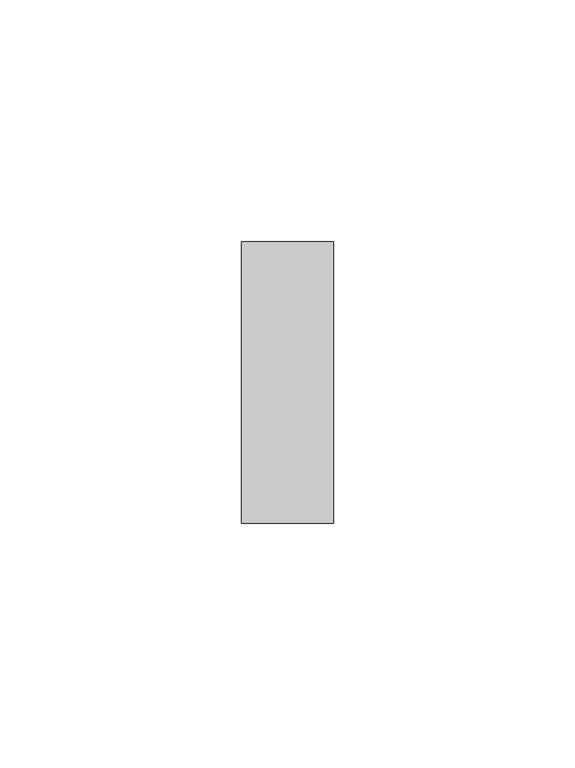
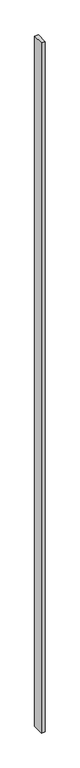
"""IFC4 building model written with IfcOpenShell, lengths in millimetres: proxy geometry, Generic Models 11:Generic Models 1:306267:Generic Models 1:306267 : Generic Models 11:Generic Models 1:306267:300405:Generic Models 1:306267:Generic Models 1:306267 : Generic Models 11:Generic Models 1:306267:300405 : Generic Models 11:Generic Models 1:306267:Generic Models 1:306267 : Generic Models 11:Generic Models 1:306267:300405:18 : Generic Models 11:Generic Models 1:306267:Generic Models 1:306267 : Generic Models 11:Generic Models 1:306267:300405:Generic Models 1:306267:Generic Models 1:306267 : Generic Models 11:Generic Models 1:306267:300405 : Generic Models 11:Generic Models 1:306267:Generic Models 1:306267 : Generic Models 11:Generic Models 1:306267:300405:300182."""

from ifc_helpers import new_model, si_unit, origin, origin_with_axes, place, context, project, spatial, polyline, outline, extrude, source, transform, mapped, element, save


def generic_models_e61006f9(model_context):
    return source(origin(), model_context, "Body", "SweptSolid", [
        extrude(outline(polyline([(596163.786724, -579018.6137729), (596182.8367239, -579018.6137729), (596182.8367239, -579076.8913841), (596163.786724, -579076.8913841), (596163.786724, -579018.6137729)])), origin_with_axes(), (0.0, 0.0, 1.0), 3689.35),
    ])


if __name__ == "__main__":
    model = new_model("IFC4")
    model_context = context("Model", 3, world=origin())
    ifc_project = project(units=[si_unit("LENGTHUNIT", "METRE", prefix="MILLI")], contexts=[model_context])
    site = spatial("IfcSite", under=ifc_project)
    building = spatial("IfcBuilding", under=site)
    placement = place(None, origin())
    generic_models_shape = generic_models_e61006f9(model_context)
    element("IfcBuildingElementProxy", 1, Name="Generic Models 11:Generic Models 1:306267:Generic Models 1:306267 : Generic Models 11:Generic Models 1:306267:300405:Generic Models 1:306267:Generic Models 1:306267 : Generic Models 11:Generic Models 1:306267:300405 : Generic Models 11:Generic Models 1:306267:Generic Models 1:306267 : Generic Models 11:Generic Models 1:306267:300405:18 : Generic Models 11:Generic Models 1:306267:Generic Models 1:306267 : Generic Models 11:Generic Models 1:306267:300405:Generic Models 1:306267:Generic Models 1:306267 : Generic Models 11:Generic Models 1:306267:300405 : Generic Models 11:Generic Models 1:306267:Generic Models 1:306267 : Generic Models 11:Generic Models 1:306267:300405:300182", ObjectType="Generic Models 11:Generic Models 1:306267:Generic Models 1:306267 : Generic Models 11:Generic Models 1:306267:300405:Generic Models 1:306267:Generic Models 1:306267 : Generic Models 11:Generic Models 1:306267:300405 : Generic Models 11:Generic Models 1:306267:Generic Models 1:306267 : Generic Models 11:Generic Models 1:306267:300405:18 : Generic Models 11:Generic Models 1:306267:Generic Models 1:306267 : Generic Models 11:Generic Models 1:306267:300405:Generic Models 1:306267:Generic Models 1:306267 : Generic Models 11:Generic Models 1:306267:300405 : Generic Models 11:Generic Models 1:306267:Generic Models 1:306267 : Generic Models 11:Generic Models 1:306267:300405:300182", at=placement, inside=building, context=model_context, shape_type="MappedRepresentation", body=[
        mapped(generic_models_shape, transform((0.0, 0.0, 0.0), x_axis=(1.0, 0.0, 0.0), y_axis=(0.0, 1.0, 0.0), z_axis=(0.0, 0.0, 1.0))),
    ])
    save(model, "model.ifc")

# Revit data of these elements
# Type "Generic Models 11:Generic Models 1:306267:Generic Models 1:306267 : Generic Models 11:Generic Models 1:306267:300405:Generic Models 1:306267:Generic Models 1:306267 : Generic Models 11:Generic Models 1:306267:300405 : Generic Models 11:Generic Models 1:306267:Generic Models 1:306267 : Generic Models 11:Generic Models 1:306267:300405:18 : Generic Models 11:Generic Models 1:306267:Generic Models 1:306267 : Generic Models 11:Generic Models 1:306267:300405:Generic Models 1:306267:Generic Models 1:306267 : Generic Models 11:Generic Models 1:306267:300405 : Generic Models 11:Generic Models 1:306267:Generic Models 1:306267 : Generic Models 11:Generic Models 1:306267:300405:300182"
#   NameOverride = "Generic Models 11:Generic Models 1:306267:Generic Models 1:306267 : Generic Models 11:Generic Models 1:306267:300405:Generic Models 1:306267:Generic Models 1:306267 : Generic Models 11:Generic Models 1:306267:300405 : Generic Models 11:Generic Models 1:306267:Generic Models 1:306267 : Generic Models 11:Generic Models 1:306267:300405:300182"
#   ObjectTypeOverride = "Generic Models 1:306267:Generic Models 1:306267 : Generic Models 11:Generic Models 1:306267:300405 : Generic Models 11:Generic Models 1:306267:Generic Models 1:306267 : Generic Models 11:Generic Models 1:306267:300405"
#   Reference = "Generic Models 1"
#   Tag = "300182"
# Element 1 (IfcBuildingElementProxy, "Generic Models 11:Generic Models 1:306267:Generic Models 1:306267 : Generic Models 11:Generic Models 1:306267:300405:Generic Models 1:306267:Generic Models 1:306267 : Generic Models 11:Generic Models 1:306267:300405 : Generic Models 11:Generic Models 1:306267:Generic Models 1:306267 : Generic Models 11:Generic Models 1:306267:300405:18 : Generic Models 11:Generic Models 1:306267:Generic Models 1:306267 : Generic Models 11:Generic Models 1:306267:300405:Generic Models 1:306267:Generic Models 1:306267 : Generic Models 11:Generic Models 1:306267:300405 : Generic Models 11:Generic Models 1:306267:Generic Models 1:306267 : Generic Models 11:Generic Models 1:306267:300405:300182")
#   Materials on its faces: "PRESSURE TREATED WOOD BLOCKING - SIZE AS NECESSARY"
# Materials
#   "PRESSURE TREATED WOOD BLOCKING - SIZE AS NECESSARY": class "Wood", colour RGB 144 113 62, transparency 0, Description = "Pinus Echinata", Cost = 0
